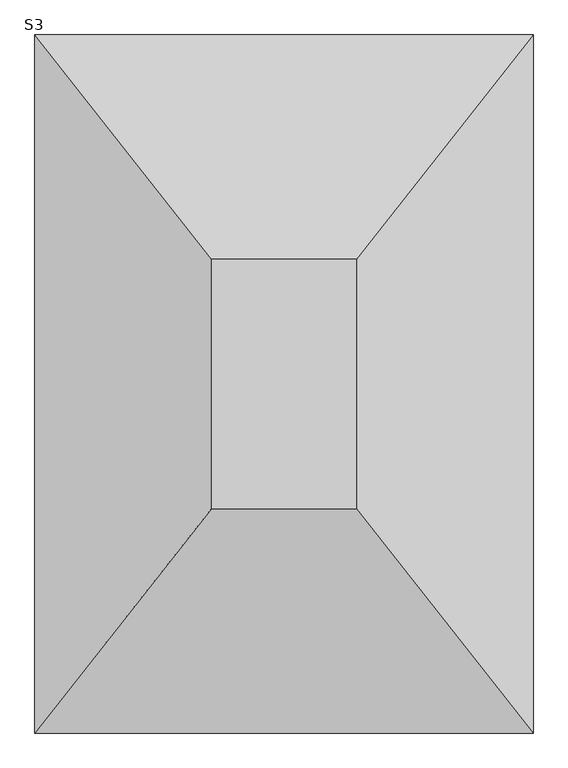
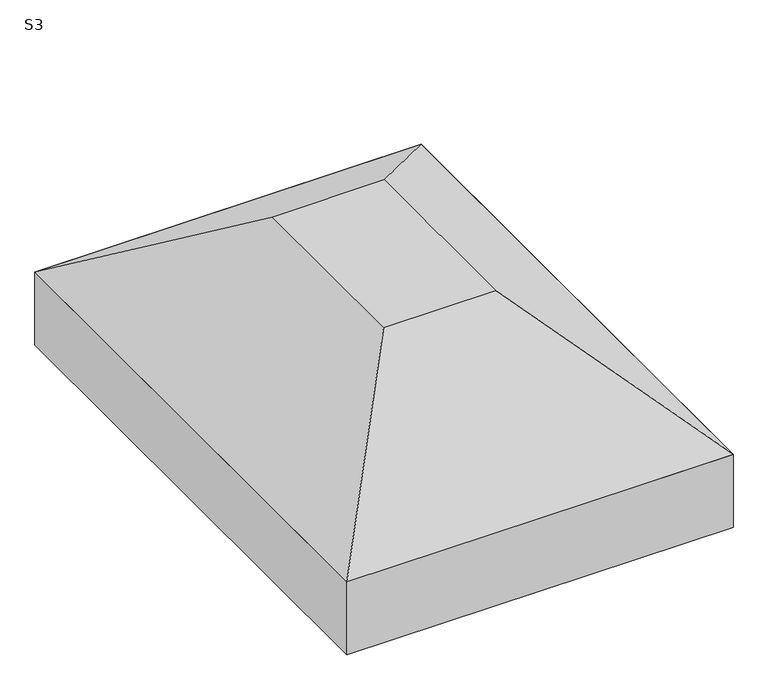
"""IFC4 building model written with IfcOpenShell, lengths in millimetres: fastener geometry, TQS - Sapata : S3."""

import ifcopenshell
import ifcopenshell.guid

model = None  # the IFC model being written
_history = None  # IfcOwnerHistory: only IFC2X3 demands one
_inside = {}  # id of a spatial element -> (the spatial element, [elements in it])
_under = {}  # id of a project, library or spatial element -> (it, [spatial elements below it])
_declared = {}  # id of a project -> (the project, [libraries it declares])
_typed = {}  # id of a type object -> (the type object, [elements of that type])
_made_of = {}  # id of a material, layer set ... -> (it, [elements and type objects made of it])


def new_model(schema):
    """Start an empty IFC model of exactly this schema.

    Asked for "IFC4X3", IfcOpenShell would pick the latest addendum, in which some entities
    have other attributes; the version numbers below select the first issue.
    IFC2X3 requires an IfcOwnerHistory on every rooted entity: one is made here for all.
    """
    global model, _history
    if schema == "IFC4X3":
        model = ifcopenshell.file(schema_version=(4, 3, 0, 0))
    else:
        model = ifcopenshell.file(schema=schema)
    _inside.clear()
    _under.clear()
    _declared.clear()
    _typed.clear()
    _made_of.clear()
    _history = None
    if model.schema == "IFC2X3":
        org = make("IfcOrganization", Name="unknown")
        user = make(
            "IfcPersonAndOrganization",
            ThePerson=make("IfcPerson", FamilyName="unknown"),
            TheOrganization=org,
        )
        app = make(
            "IfcApplication",
            ApplicationDeveloper=org,
            Version="unknown",
            ApplicationFullName="unknown",
            ApplicationIdentifier="unknown",
        )
        _history = make(
            "IfcOwnerHistory",
            OwningUser=user,
            OwningApplication=app,
            ChangeAction="ADDED",
            CreationDate=0,
        )
    return model


def make(cls, **values):
    """One entity of the class cls with the attributes given. An attribute that is None is left unset."""
    return model.create_entity(
        cls, **{name: value for name, value in values.items() if value is not None}
    )


def rooted(cls, **values):
    """An entity with a GlobalId (a new one), such as an element, a storey or a relation."""
    return make(cls, GlobalId=ifcopenshell.guid.new(), OwnerHistory=_history, **values)


def si_unit(unit_type, name, prefix=None):
    """IfcSIUnit, for example si_unit("LENGTHUNIT", "METRE", prefix="MILLI")."""
    return make("IfcSIUnit", UnitType=unit_type, Prefix=prefix, Name=name)


def assignment(units):
    """IfcUnitAssignment: the units of a project."""
    return None if units is None else make("IfcUnitAssignment", Units=units)


def point(xyz):
    """IfcCartesianPoint."""
    return None if xyz is None else make("IfcCartesianPoint", Coordinates=xyz)


def direction(xyz):
    """IfcDirection."""
    return None if xyz is None else make("IfcDirection", DirectionRatios=xyz)


def frame(location, z_axis=None, x_axis=None):
    """IfcAxis2Placement3D, a coordinate frame: its origin and axes. An axis left out is left unset."""
    return make(
        "IfcAxis2Placement3D",
        Location=point(location),
        Axis=direction(z_axis),
        RefDirection=direction(x_axis),
    )


def origin():
    """The frame at (0, 0, 0) with its axes left unset."""
    return frame((0.0, 0.0, 0.0))


def place(relative_to, where):
    """IfcLocalPlacement: puts the frame where relative to a parent placement (None: the world)."""
    return make(
        "IfcLocalPlacement", PlacementRelTo=relative_to, RelativePlacement=where
    )


def context(
    kind, dimensions, precision=None, world=None, true_north=None, identifier=None
):
    """IfcGeometricRepresentationContext, for example the 3D "Model" context."""
    return make(
        "IfcGeometricRepresentationContext",
        ContextIdentifier=identifier,
        ContextType=kind,
        CoordinateSpaceDimension=dimensions,
        Precision=precision,
        WorldCoordinateSystem=world,
        TrueNorth=true_north,
    )


def project(units=None, contexts=None):
    """IfcProject with its units and contexts."""
    return rooted(
        "IfcProject",
        Name="project",
        RepresentationContexts=contexts,
        UnitsInContext=assignment(units),
    )


def spatial(cls, under=None, at=None, **own):
    """A site, building, storey or space (cls), placed at a placement, below another one or the project."""
    s = rooted(cls, ObjectPlacement=at, **own)
    if under is not None:
        _under.setdefault(under.id(), (under, []))[1].append(s)
    return s


def polyline(points):
    """IfcPolyline through the points."""
    return make("IfcPolyline", Points=[point(p) for p in points])


def outline(outer, holes=None, kind="AREA"):
    """IfcArbitraryClosedProfileDef: a profile drawn as a closed curve; with holes, ...WithVoids."""
    if holes is None:
        return make("IfcArbitraryClosedProfileDef", ProfileType=kind, OuterCurve=outer)
    return make(
        "IfcArbitraryProfileDefWithVoids",
        ProfileType=kind,
        OuterCurve=outer,
        InnerCurves=holes,
    )


def extrude(swept, where, along, depth):
    """IfcExtrudedAreaSolid: the profile swept, set in the frame where, extruded along a direction by depth."""
    return make(
        "IfcExtrudedAreaSolid",
        SweptArea=swept,
        Position=where,
        ExtrudedDirection=direction(along),
        Depth=depth,
    )


def faces_of(points, faces, orient=None, outer=None):
    """IfcFace entities. A face is a list of loops; a loop is a list of indices into points, from 0.

    orient and outer hold one flag for each loop. By default every Orientation is true, the
    first loop of a face is its IfcFaceOuterBound and the others are IfcFaceBound.
    """
    made = []
    for i, loops in enumerate(faces):
        bounds = []
        for j, loop in enumerate(loops):
            is_outer = j == 0 if outer is None else outer[i][j]
            bounds.append(
                make(
                    "IfcFaceOuterBound" if is_outer else "IfcFaceBound",
                    Bound=make("IfcPolyLoop", Polygon=[points[k] for k in loop]),
                    Orientation=True if orient is None else orient[i][j],
                )
            )
        made.append(make("IfcFace", Bounds=bounds))
    return made


def faceted_brep(points, faces, orient=None, outer=None, voids=None):
    """IfcFacetedBrep: a solid bounded by flat faces; with voids (closed shells), ...WithVoids."""
    shared = [point(p) for p in points]
    hull = make("IfcClosedShell", CfsFaces=faces_of(shared, faces, orient, outer))
    if voids is None:
        return make("IfcFacetedBrep", Outer=hull)
    return make(
        "IfcFacetedBrepWithVoids",
        Outer=hull,
        Voids=[
            make(cls, CfsFaces=faces_of(shared, fs, o, b)) for cls, fs, o, b in voids
        ],
    )


def shape(context_of_items, identifier, shape_type, items):
    """IfcShapeRepresentation: the items that make up one representation, for example the "Body"."""
    return make(
        "IfcShapeRepresentation",
        ContextOfItems=context_of_items,
        RepresentationIdentifier=identifier,
        RepresentationType=shape_type,
        Items=items,
    )


def source(mapping_origin, context_of_items, identifier, shape_type, items):
    """IfcRepresentationMap: a shape defined once, which mapped items show again and again."""
    return make(
        "IfcRepresentationMap",
        MappingOrigin=mapping_origin,
        MappedRepresentation=shape(context_of_items, identifier, shape_type, items),
    )


def transform(
    local_origin,
    x_axis=None,
    y_axis=None,
    z_axis=None,
    scale=None,
    scale2=None,
    scale3=None,
    uniform=True,
):
    """IfcCartesianTransformationOperator3D, or its non-uniform kind. x_axis, y_axis, z_axis: its Axis1, 2, 3."""
    if uniform:
        return make(
            "IfcCartesianTransformationOperator3D",
            Axis1=direction(x_axis),
            Axis2=direction(y_axis),
            LocalOrigin=point(local_origin),
            Scale=scale,
            Axis3=direction(z_axis),
        )
    return make(
        "IfcCartesianTransformationOperator3DnonUniform",
        Axis1=direction(x_axis),
        Axis2=direction(y_axis),
        LocalOrigin=point(local_origin),
        Scale=scale,
        Axis3=direction(z_axis),
        Scale2=scale2,
        Scale3=scale3,
    )


def mapped(mapping_source, mapping_target):
    """IfcMappedItem: shows the shape of a source again, moved by a transform."""
    return make(
        "IfcMappedItem", MappingSource=mapping_source, MappingTarget=mapping_target
    )


def made_of(thing, what):
    """Note that an element or type object is made of a material, layer set ...; save() writes the relation."""
    if what is not None:
        _made_of.setdefault(what.id(), (what, []))[1].append(thing)
    return thing


def element(
    cls,
    number,
    at=None,
    inside=None,
    cuts=None,
    type_object=None,
    material=None,
    context=None,
    identifier="Body",
    shape_type=None,
    held_by="IfcProductDefinitionShape",
    body=None,
    shapes=None,
    **own,
):
    """One element of the class cls, such as IfcWall. Its Tag is "e" and its number.

    at: its placement. inside: the storey or other place that contains it. cuts: it is an
    opening in that element (IfcRelVoidsElement). A single representation is given by context,
    identifier, shape_type and body (its items); several are given by shapes. held_by: the class
    of the entity that holds the representations. save() writes the other relations.
    """
    e = rooted(cls, Tag="e%d" % number, ObjectPlacement=at, **own)
    if body is not None:
        shapes = [shape(context, identifier, shape_type, body)]
    if shapes is not None:
        e.Representation = make(held_by, Representations=shapes)
    if inside is not None:
        _inside.setdefault(inside.id(), (inside, []))[1].append(e)
    if cuts is not None:
        rooted(
            "IfcRelVoidsElement", RelatingBuildingElement=cuts, RelatedOpeningElement=e
        )
    if type_object is not None:
        _typed.setdefault(type_object.id(), (type_object, []))[1].append(e)
    return made_of(e, material)


def aggregate(whole, parts):
    """IfcRelAggregates: a whole, such as a stair, and the parts it consists of."""
    return rooted("IfcRelAggregates", RelatingObject=whole, RelatedObjects=parts)


def save(model, path):
    """Write the relations noted so far, then the file.

    IfcRelAggregates (storeys below a building ...), IfcRelContainedInSpatialStructure (elements
    in a storey), IfcRelDefinesByType, IfcRelAssociatesMaterial and IfcRelDeclares: one each for
    every whole, place, type object, material and project.
    """
    for whole, parts in _under.values():
        aggregate(whole, parts)
    for where, things in _inside.values():
        rooted(
            "IfcRelContainedInSpatialStructure",
            RelatedElements=things,
            RelatingStructure=where,
        )
    for kind, things in _typed.values():
        rooted("IfcRelDefinesByType", RelatedObjects=things, RelatingType=kind)
    for what, things in _made_of.values():
        rooted("IfcRelAssociatesMaterial", RelatedObjects=things, RelatingMaterial=what)
    for by, libraries in _declared.values():
        rooted("IfcRelDeclares", RelatingContext=by, RelatedDefinitions=libraries)
    model.write(path)


def s3_fc183e28(model_context):
    return source(origin(), model_context, "Body", "SolidModel", [
        faceted_brep([(-55.0, 50.0, 0.0), (-345.0, 50.0, 0.0), (-345.0, -450.0, 0.0), (-55.0, -450.0, 0.0), (300.0, 500.0, -300.0), (300.0, -900.0, -300.0), (-700.0, -900.0, -300.0), (-700.0, 500.0, -300.0)], [[[0, 1, 2, 3]], [[4, 5, 6, 7]], [[4, 7, 1, 0]], [[7, 6, 2, 1]], [[6, 5, 3, 2]], [[5, 4, 0, 3]]]),
        extrude(outline(polyline([(300.0, 500.0), (300.0, -900.0), (-700.0, -900.0), (-700.0, 500.0), (300.0, 500.0)])), frame((0.0, 0.0, -500.0), z_axis=(0.0, 0.0, 1.0), x_axis=(1.0, 0.0, 0.0)), (0.0, 0.0, 1.0), 200.0),
    ])


if __name__ == "__main__":
    model = new_model("IFC4")
    model_context = context("Model", 3, world=origin())
    ifc_project = project(units=[si_unit("LENGTHUNIT", "METRE", prefix="MILLI")], contexts=[model_context])
    site = spatial("IfcSite", under=ifc_project)
    building = spatial("IfcBuilding", under=site)
    placement = place(None, origin())
    s3_shape = s3_fc183e28(model_context)
    element("IfcFastener", 1, ObjectType="TQS - Sapata : S3", at=placement, inside=building, context=model_context, shape_type="MappedRepresentation", body=[
        mapped(s3_shape, transform((0.0, 0.0, 0.0), x_axis=(1.0, 0.0, 0.0), y_axis=(0.0, 1.0, 0.0), z_axis=(0.0, 0.0, 1.0))),
    ])
    save(model, "model.ifc")

# Revit data of these elements
# Type "TQS - Sapata : S3"
#   TY = 0.50 m
#   TX = 0.29 m
#   HS = 0.50 m
#   H0 = 0.20 m
#   EXCYABS = 0.70 m
#   EXCY = 0.00 m
#   EXCXABS = 0.50 m
#   EXCX = 0.00 m
#   DIMY = 1.40 m
#   DIMX = 1.00 m
#   Material estrutural = Concreto - Concreto concretado no local
#   Width = 0
#   Length = 0
# Element 1 (IfcFastener, "TQS - Sapata : S3")
#   Materials on its faces: "Concreto - Concreto concretado no local"
# Materials
#   "Concreto - Concreto concretado no local": class "Concreto", colour RGB 192 192 192, transparency 0
